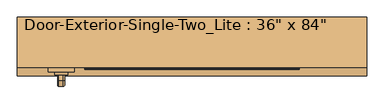
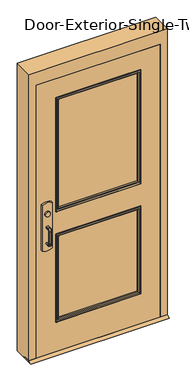
"""IFC4 building model written with IfcOpenShell, lengths in millimetres: door geometry."""

from ifc_helpers import new_model, si_unit, point, frame, frame_2d, origin, place, context, project, spatial, polyline, circle_curve, ellipse_curve, trimmed, segment, composite_curve, outline, extrude, faceted_brep, source, transform, mapped, element, save
from ifc_brep_helpers import plane_surface, cylinder_surface, revolved_surface, advanced_brep


def door_0d86e27c(model_context):
    return source(origin(), model_context, "Body", "SolidModel", [
        extrude(outline(polyline([(-61.9125, 12.7), (-36.5125, 0.0), (-131.7625, 0.0), (-106.3625, 12.7), (-61.9125, 12.7)])), frame((-508.0, 0.0, 0.0), z_axis=(1.0, 0.0, 0.0), x_axis=(0.0, 1.0, 0.0)), (0.0, 0.0, 1.0), 1016.0),
        extrude(outline(polyline([(150.2833333, -23.8125), (150.2833333, -30.1625), (-349.25, -30.1625), (-349.25, -23.8125), (150.2833333, -23.8125)])), frame((0.0, 0.0, 990.6), z_axis=(0.0, 0.0, 1.0), x_axis=(1.0, 0.0, 0.0)), (0.0, 0.0, 1.0), 50.8),
        advanced_brep(
        [(-412.75, -30.1625, 1041.4), (-349.25, -30.1625, 1041.4), (400.05, -30.1625, 1041.4), (400.05, -30.1625, 990.6), (-349.25, -30.1625, 990.6), (-412.75, -30.1625, 990.6), (400.05, -61.9125, 1041.4), (-349.25, -61.9125, 1041.4), (-349.25, -61.9125, 1104.9), (-368.3, -61.9125, 1123.95), (-393.7, -61.9125, 1123.95), (-412.75, -61.9125, 1104.9), (-412.75, -61.9125, 927.1), (-393.7, -61.9125, 908.05), (-368.3, -61.9125, 908.05), (-349.25, -61.9125, 927.1), (-349.25, -61.9125, 990.6), (400.05, -61.9125, 990.6), (-412.75, -33.3377467, 1041.4), (-349.25, -33.3377467, 1041.4), (-412.75, -33.3377467, 990.6), (-412.75, -38.3479269, 927.1), (-412.75, -38.3479269, 1104.9), (-349.25, -33.3377467, 990.6), (-349.25, -38.3479269, 1104.9), (-349.25, -38.3479269, 927.1), (-368.3, -39.850981, 1123.95), (-393.7, -39.850981, 1123.95), (-393.7, -39.850981, 908.05), (-368.3, -39.850981, 908.05)],
        [
            (0, 1),
            (1, 2),
            (2, 3),
            (3, 4),
            (4, 5),
            (5, 0),
            (6, 7),
            (7, 8),
            (8, 9, circle_curve(frame((-368.3, -61.9125, 1104.9), z_axis=(0.0, -1.0, 0.0), x_axis=(1.0, 0.0, 0.0)), 19.05)),
            (9, 10),
            (10, 11, circle_curve(frame((-393.7, -61.9125, 1104.9), z_axis=(0.0, -1.0, 0.0), x_axis=(1.0, 0.0, 0.0)), 19.05)),
            (11, 12),
            (12, 13, circle_curve(frame((-393.7, -61.9125, 927.1), z_axis=(0.0, -1.0, 0.0), x_axis=(1.0, 0.0, 0.0)), 19.05)),
            (13, 14),
            (14, 15, circle_curve(frame((-368.3, -61.9125, 927.1), z_axis=(0.0, -1.0, 0.0), x_axis=(1.0, 0.0, 0.0)), 19.05)),
            (15, 16),
            (16, 17),
            (17, 6),
            (0, 18),
            (18, 19),
            (19, 7),
            (6, 2),
            (5, 20),
            (20, 21),
            (21, 12),
            (11, 22),
            (22, 18),
            (16, 23),
            (23, 20),
            (3, 17),
            (19, 24),
            (24, 8),
            (15, 25),
            (25, 23),
            (9, 26),
            (26, 27),
            (27, 10),
            (13, 28),
            (28, 29),
            (29, 14),
            (29, 25, ellipse_curve(frame((-368.3, -38.3479269, 927.1), z_axis=(0.0, -0.9969018152893365, 0.07865602756830282), x_axis=(0.0, 0.07865602756830208, 0.9969018152893365)), 19.1092038, 19.05)),
            (24, 26, ellipse_curve(frame((-368.3, -38.3479269, 1104.9), z_axis=(0.0, -0.9969018152893376, -0.07865602756828934), x_axis=(0.0, 0.078656027568288, -0.9969018152893377)), 19.1092038, 19.05)),
            (27, 22, ellipse_curve(frame((-393.7, -38.3479269, 1104.9), z_axis=(0.0, -0.9969018152893376, -0.07865602756828934), x_axis=(0.0, 0.078656027568288, -0.9969018152893377)), 19.1092038, 19.05)),
            (21, 28, ellipse_curve(frame((-393.7, -38.3479269, 927.1), z_axis=(0.0, -0.9969018152893365, 0.07865602756830282), x_axis=(0.0, 0.07865602756830208, 0.9969018152893365)), 19.1092038, 19.05)),
        ],
        [
            plane_surface(frame((-412.75, -30.1625, 1041.4), z_axis=(0.0, 1.0, 0.0), x_axis=(-1.0, 0.0, 0.0))),
            plane_surface(frame((-412.75, -61.9125, 1041.4), z_axis=(0.0, -1.0, 0.0), x_axis=(1.0, 0.0, 0.0))),
            plane_surface(frame((400.05, -30.1625, 1041.4), z_axis=(0.0, 0.0, 1.0), x_axis=(0.0, -1.0, 0.0))),
            plane_surface(frame((-412.75, -30.1625, 1041.4), z_axis=(-1.0, 0.0, 0.0), x_axis=(0.0, -1.0, 0.0))),
            plane_surface(frame((-412.75, -30.1625, 990.6), z_axis=(0.0, 0.0, -1.0), x_axis=(0.0, -1.0, 0.0))),
            plane_surface(frame((400.05, -30.1625, 990.6), z_axis=(1.0, 0.0, 0.0), x_axis=(0.0, -1.0, 0.0))),
            plane_surface(frame((-349.25, -33.3377467, 927.1), z_axis=(1.0, 0.0, 0.0), x_axis=(0.0, -1.0, 0.0))),
            plane_surface(frame((-368.3, -33.3377467, 1123.95), z_axis=(0.0, 0.0, 1.0), x_axis=(0.0, -1.0, 0.0))),
            plane_surface(frame((-393.7, -33.3377467, 908.05), z_axis=(0.0, 0.0, -1.0), x_axis=(0.0, -1.0, 0.0))),
            cylinder_surface(frame((-368.3, -61.9125, 927.1), z_axis=(0.0, 1.0, 0.0), x_axis=(1.0, 0.0, 0.0)), 19.05),
            cylinder_surface(frame((-368.3, -61.9125, 1104.9), z_axis=(0.0, 1.0, 0.0), x_axis=(1.0, 0.0, 0.0)), 19.05),
            cylinder_surface(frame((-393.7, -61.9125, 1104.9), z_axis=(0.0, 1.0, 0.0), x_axis=(1.0, 0.0, 0.0)), 19.05),
            cylinder_surface(frame((-393.7, -61.9125, 927.1), z_axis=(0.0, 1.0, 0.0), x_axis=(1.0, 0.0, 0.0)), 19.05),
            plane_surface(frame((-349.25, -33.3377467, 1041.4), z_axis=(0.0, 0.9969018152893376, 0.07865602756828934), x_axis=(-1.0, 0.0, 0.0))),
            plane_surface(frame((-349.25, -39.850981, 908.05), z_axis=(0.0, 0.9969018152893365, -0.07865602756830282), x_axis=(-1.0, 0.0, 0.0))),
        ],
        [
            (0, [[1, 2, 3, 4, 5, 6]]),
            (1, [[7, 8, 9, 10, 11, 12, 13, 14, 15, 16, 17, 18]]),
            (2, [[-2, -1, 19, 20, 21, -7, 22]]),
            (3, [[23, 24, 25, -12, 26, 27, -19, -6]]),
            (4, [[-17, 28, 29, -23, -5, -4, 30]]),
            (5, [[-22, -18, -30, -3]]),
            (6, [[-21, 31, 32, -8]]),
            (6, [[33, 34, -28, -16]]),
            (7, [[35, 36, 37, -10]]),
            (8, [[38, 39, 40, -14]]),
            (9, [[-40, 41, -33, -15]]),
            (10, [[-32, 42, -35, -9]]),
            (11, [[-37, 43, -26, -11]]),
            (12, [[-25, 44, -38, -13]]),
            (13, [[-27, -43, -36, -42, -31, -20]]),
            (14, [[-29, -34, -41, -39, -44, -24]]),
        ],
    ),
        advanced_brep(
        [(-391.0, -119.0625, 1017.190625), (-387.428125, -119.0625, 1020.7625), (-374.571875, -119.0625, 1020.7625), (-371.0, -119.0625, 1017.190625), (-371.0, -119.0625, 1014.8090406), (-374.5715406, -119.0625, 1011.2375), (-387.428125, -119.0625, 1011.2375), (-391.0, -119.0625, 1014.809375), (-391.0, -119.0625, 887.809375), (-391.0, -119.0625, 890.190625), (-387.428125, -119.0625, 893.7625), (-374.5715406, -119.0625, 893.7625), (-371.0, -119.0625, 890.1909594), (-371.0, -119.0625, 887.809375), (-374.571875, -119.0625, 884.2375), (-387.428125, -119.0625, 884.2375), (-391.0, -144.4625, 1014.809375), (-391.0, -155.971875, 1003.3), (-391.0, -155.971875, 901.7), (-391.0, -144.4625, 890.190625), (-391.0, -144.4625, 887.809375), (-391.0, -158.353125, 901.7), (-391.0, -158.353125, 1003.3), (-391.0, -144.4625, 1017.190625), (-387.428125, -144.4625, 1011.2375), (-374.5715406, -144.4625, 1011.2375), (-371.0, -144.4625, 1014.8090406), (-371.0, -144.4625, 1017.190625), (-371.0, -158.353125, 1003.3), (-371.0, -158.353125, 901.7), (-371.0, -144.4625, 887.809375), (-371.0, -144.4625, 890.1909594), (-371.0, -155.9715406, 901.7), (-371.0, -155.9715406, 1003.3), (-374.571875, -144.4625, 1020.7625), (-387.428125, -144.4625, 1020.7625), (-387.428125, -152.4, 1003.3), (-374.5715406, -152.4, 1003.3), (-374.571875, -161.925, 1003.3), (-387.428125, -161.925, 1003.3), (-387.428125, -152.4, 901.7), (-374.5715406, -152.4, 901.7), (-374.571875, -161.925, 901.7), (-387.428125, -161.925, 901.7), (-387.428125, -144.4625, 893.7625), (-374.5715406, -144.4625, 893.7625), (-374.571875, -144.4625, 884.2375), (-387.428125, -144.4625, 884.2375)],
        [
            (0, 1, circle_curve(frame((-387.428125, -119.0625, 1017.190625), z_axis=(0.0, 1.0, 0.0), x_axis=(0.0, 0.0, 1.0)), 3.571875)),
            (1, 2),
            (2, 3, circle_curve(frame((-374.571875, -119.0625, 1017.190625), z_axis=(0.0, 1.0, 0.0), x_axis=(0.0, 0.0, 1.0)), 3.571875)),
            (3, 4),
            (4, 5, circle_curve(frame((-374.5715406, -119.0625, 1014.8090406), z_axis=(0.0, 1.0, 0.0), x_axis=(0.0, 0.0, 1.0)), 3.5715406)),
            (5, 6),
            (6, 7, circle_curve(frame((-387.428125, -119.0625, 1014.809375), z_axis=(0.0, 1.0, 0.0), x_axis=(0.0, 0.0, 1.0)), 3.571875)),
            (7, 0),
            (8, 9),
            (9, 10, circle_curve(frame((-387.428125, -119.0625, 890.190625), z_axis=(0.0, 1.0, 0.0), x_axis=(0.0, 0.0, -1.0)), 3.571875)),
            (10, 11),
            (11, 12, circle_curve(frame((-374.5715406, -119.0625, 890.1909594), z_axis=(0.0, 1.0, 0.0), x_axis=(0.0, 0.0, -1.0)), 3.5715406)),
            (12, 13),
            (13, 14, circle_curve(frame((-374.571875, -119.0625, 887.809375), z_axis=(0.0, 1.0, 0.0), x_axis=(0.0, 0.0, -1.0)), 3.571875)),
            (14, 15),
            (15, 8, circle_curve(frame((-387.428125, -119.0625, 887.809375), z_axis=(0.0, 1.0, 0.0), x_axis=(0.0, 0.0, -1.0)), 3.571875)),
            (7, 16),
            (16, 17, circle_curve(frame((-391.0, -144.4625, 1003.3), z_axis=(1.0, 0.0, 0.0), x_axis=(0.0, 0.0, 1.0)), 11.509375)),
            (17, 18),
            (18, 19, circle_curve(frame((-391.0, -144.4625, 901.7), z_axis=(1.0, 0.0, 0.0), x_axis=(0.0, -1.0, 0.0)), 11.509375)),
            (19, 9),
            (8, 20),
            (20, 21, circle_curve(frame((-391.0, -144.4625, 901.7), z_axis=(-1.0, 0.0, 0.0), x_axis=(0.0, -1.0, 0.0)), 13.890625)),
            (21, 22),
            (22, 23, circle_curve(frame((-391.0, -144.4625, 1003.3), z_axis=(-1.0, 0.0, 0.0), x_axis=(0.0, 0.0, 1.0)), 13.890625)),
            (23, 0),
            (6, 24),
            (24, 16, circle_curve(frame((-387.428125, -144.4625, 1014.809375), z_axis=(0.0, 1.0, 0.0), x_axis=(0.0, 0.0, 1.0)), 3.571875)),
            (5, 25),
            (25, 24),
            (4, 26),
            (26, 25, circle_curve(frame((-374.5715406, -144.4625, 1014.8090406), z_axis=(0.0, 1.0, 0.0), x_axis=(0.0, 0.0, 1.0)), 3.5715406)),
            (3, 27),
            (27, 28, circle_curve(frame((-371.0, -144.4625, 1003.3), z_axis=(1.0, 0.0, 0.0), x_axis=(0.0, 0.0, 1.0)), 13.890625)),
            (28, 29),
            (29, 30, circle_curve(frame((-371.0, -144.4625, 901.7), z_axis=(1.0, 0.0, 0.0), x_axis=(0.0, -1.0, 0.0)), 13.890625)),
            (30, 13),
            (12, 31),
            (31, 32, circle_curve(frame((-371.0, -144.4625, 901.7), z_axis=(-1.0, 0.0, 0.0), x_axis=(0.0, -1.0, 0.0)), 11.5090406)),
            (32, 33),
            (33, 26, circle_curve(frame((-371.0, -144.4625, 1003.3), z_axis=(-1.0, 0.0, 0.0), x_axis=(0.0, 0.0, 1.0)), 11.5090406)),
            (2, 34),
            (34, 27, circle_curve(frame((-374.571875, -144.4625, 1017.190625), z_axis=(0.0, 1.0, 0.0), x_axis=(0.0, 0.0, 1.0)), 3.571875)),
            (1, 35),
            (35, 34),
            (23, 35, circle_curve(frame((-387.428125, -144.4625, 1017.190625), z_axis=(0.0, 1.0, 0.0), x_axis=(0.0, 0.0, 1.0)), 3.571875)),
            (36, 17, circle_curve(frame((-387.428125, -155.971875, 1003.3), z_axis=(0.0, 0.0, 1.0), x_axis=(0.0, -1.0, 0.0)), 3.571875)),
            (24, 36, circle_curve(frame((-387.428125, -144.4625, 1003.3), z_axis=(1.0, 0.0, 0.0), x_axis=(0.0, 0.0, 1.0)), 7.9375)),
            (37, 36),
            (25, 37, circle_curve(frame((-374.5715406, -144.4625, 1003.3), z_axis=(1.0, 0.0, 0.0), x_axis=(0.0, 0.0, 1.0)), 7.9375)),
            (33, 37, circle_curve(frame((-374.5715406, -155.9715406, 1003.3), z_axis=(0.0, 0.0, 1.0), x_axis=(0.0, -1.0, 0.0)), 3.5715406)),
            (38, 28, circle_curve(frame((-374.571875, -158.353125, 1003.3), z_axis=(0.0, 0.0, 1.0), x_axis=(0.0, -1.0, 0.0)), 3.571875)),
            (34, 38, circle_curve(frame((-374.571875, -144.4625, 1003.3), z_axis=(1.0, 0.0, 0.0), x_axis=(0.0, 0.0, 1.0)), 17.4625)),
            (39, 38),
            (35, 39, circle_curve(frame((-387.428125, -144.4625, 1003.3), z_axis=(1.0, 0.0, 0.0), x_axis=(0.0, 0.0, 1.0)), 17.4625)),
            (22, 39, circle_curve(frame((-387.428125, -158.353125, 1003.3), z_axis=(0.0, 0.0, 1.0), x_axis=(0.0, -1.0, 0.0)), 3.571875)),
            (36, 40),
            (40, 18, circle_curve(frame((-387.428125, -155.971875, 901.7), z_axis=(0.0, 0.0, 1.0), x_axis=(0.0, -1.0, 0.0)), 3.571875)),
            (37, 41),
            (41, 40),
            (32, 41, circle_curve(frame((-374.5715406, -155.9715406, 901.7), z_axis=(0.0, 0.0, 1.0), x_axis=(0.0, -1.0, 0.0)), 3.5715406)),
            (38, 42),
            (42, 29, circle_curve(frame((-374.571875, -158.353125, 901.7), z_axis=(0.0, 0.0, 1.0), x_axis=(0.0, -1.0, 0.0)), 3.571875)),
            (39, 43),
            (43, 42),
            (21, 43, circle_curve(frame((-387.428125, -158.353125, 901.7), z_axis=(0.0, 0.0, 1.0), x_axis=(0.0, -1.0, 0.0)), 3.571875)),
            (44, 19, circle_curve(frame((-387.428125, -144.4625, 890.190625), z_axis=(0.0, -1.0, 0.0), x_axis=(0.0, 0.0, -1.0)), 3.571875)),
            (40, 44, circle_curve(frame((-387.428125, -144.4625, 901.7), z_axis=(1.0, 0.0, 0.0), x_axis=(0.0, -1.0, 0.0)), 7.9375)),
            (45, 44),
            (41, 45, circle_curve(frame((-374.5715406, -144.4625, 901.7), z_axis=(1.0, 0.0, 0.0), x_axis=(0.0, -1.0, 0.0)), 7.9375)),
            (31, 45, circle_curve(frame((-374.5715406, -144.4625, 890.1909594), z_axis=(0.0, -1.0, 0.0), x_axis=(0.0, 0.0, -1.0)), 3.5715406)),
            (46, 30, circle_curve(frame((-374.571875, -144.4625, 887.809375), z_axis=(0.0, -1.0, 0.0), x_axis=(0.0, 0.0, -1.0)), 3.571875)),
            (42, 46, circle_curve(frame((-374.571875, -144.4625, 901.7), z_axis=(1.0, 0.0, 0.0), x_axis=(0.0, -1.0, 0.0)), 17.4625)),
            (47, 46),
            (43, 47, circle_curve(frame((-387.428125, -144.4625, 901.7), z_axis=(1.0, 0.0, 0.0), x_axis=(0.0, -1.0, 0.0)), 17.4625)),
            (20, 47, circle_curve(frame((-387.428125, -144.4625, 887.809375), z_axis=(0.0, -1.0, 0.0), x_axis=(0.0, 0.0, -1.0)), 3.571875)),
            (44, 10),
            (45, 11),
            (46, 14),
            (47, 15),
        ],
        [
            plane_surface(frame((-381.0, -119.0625, 1016.0), z_axis=(0.0, 1.0, 0.0), x_axis=(1.0, 0.0, 0.0))),
            plane_surface(frame((-381.0, -119.0625, 889.0), z_axis=(0.0, 1.0, 0.0), x_axis=(1.0, 0.0, 0.0))),
            plane_surface(frame((-391.0, -119.0625, 1017.190625), z_axis=(-1.0, 0.0, 0.0), x_axis=(0.0, -1.0, 0.0))),
            cylinder_surface(frame((-387.428125, -119.0625, 1014.809375), z_axis=(0.0, 1.0, 0.0), x_axis=(0.0, 0.0, 1.0)), 3.571875),
            plane_surface(frame((-387.428125, -119.0625, 1011.2375), z_axis=(0.0, 0.0, -1.0), x_axis=(0.0, -1.0, 0.0))),
            cylinder_surface(frame((-374.5715406, -119.0625, 1014.8090406), z_axis=(0.0, 1.0, 0.0), x_axis=(0.0, 0.0, 1.0)), 3.5715406),
            plane_surface(frame((-371.0, -119.0625, 1014.8090406), z_axis=(1.0, 0.0, 0.0), x_axis=(0.0, -1.0, 0.0))),
            cylinder_surface(frame((-374.571875, -119.0625, 1017.190625), z_axis=(0.0, 1.0, 0.0), x_axis=(0.0, 0.0, 1.0)), 3.571875),
            plane_surface(frame((-374.571875, -119.0625, 1020.7625), z_axis=(0.0, 0.0, 1.0), x_axis=(0.0, -1.0, 0.0))),
            cylinder_surface(frame((-387.428125, -119.0625, 1017.190625), z_axis=(0.0, 1.0, 0.0), x_axis=(0.0, 0.0, 1.0)), 3.571875),
            revolved_surface(trimmed(ellipse_curve(frame((-387.428125, -144.4625, 1014.809375), z_axis=(0.0, -1.0, 0.0), x_axis=(0.0, 0.0, 1.0)), 3.571875, 3.571875), [point((-391.0, -144.4625, 1014.809375))], [point((-387.428125, -144.4625, 1011.2375))], True, "CARTESIAN"), (-381.0, -144.4625, 1003.3), (-1.0, 0.0, 0.0)),
            revolved_surface(polyline([(-387.428125, -144.4625, 1011.2375), (-374.5715406, -144.4625, 1011.2375)]), (-381.0, -144.4625, 1003.3), (-1.0, 0.0, 0.0)),
            revolved_surface(trimmed(ellipse_curve(frame((-374.5715406, -144.4625, 1014.8090406), z_axis=(0.0, -1.0, 0.0), x_axis=(0.0, 0.0, 1.0)), 3.5715406, 3.5715406), [point((-374.5715406, -144.4625, 1011.2375))], [point((-371.0, -144.4625, 1014.8090406))], True, "CARTESIAN"), (-381.0, -144.4625, 1003.3), (-1.0, 0.0, 0.0)),
            revolved_surface(trimmed(ellipse_curve(frame((-374.571875, -144.4625, 1017.190625), z_axis=(0.0, -1.0, 0.0), x_axis=(0.0, 0.0, 1.0)), 3.571875, 3.571875), [point((-371.0, -144.4625, 1017.190625))], [point((-374.571875, -144.4625, 1020.7625))], True, "CARTESIAN"), (-381.0, -144.4625, 1003.3), (-1.0, 0.0, 0.0)),
            cylinder_surface(frame((-381.0, -144.4625, 1003.3), z_axis=(-1.0, 0.0, 0.0), x_axis=(0.0, 0.0, 1.0)), 17.4625),
            revolved_surface(trimmed(ellipse_curve(frame((-387.428125, -144.4625, 1017.190625), z_axis=(0.0, -1.0, 0.0), x_axis=(0.0, 0.0, 1.0)), 3.571875, 3.571875), [point((-387.428125, -144.4625, 1020.7625))], [point((-391.0, -144.4625, 1017.190625))], True, "CARTESIAN"), (-381.0, -144.4625, 1003.3), (-1.0, 0.0, 0.0)),
            cylinder_surface(frame((-387.428125, -155.971875, 1003.3), z_axis=(0.0, 0.0, 1.0), x_axis=(0.0, -1.0, 0.0)), 3.571875),
            plane_surface(frame((-387.428125, -152.4, 1003.3), z_axis=(0.0, 1.0, 0.0), x_axis=(0.0, 0.0, -1.0))),
            cylinder_surface(frame((-374.5715406, -155.9715406, 1003.3), z_axis=(0.0, 0.0, 1.0), x_axis=(0.0, -1.0, 0.0)), 3.5715406),
            cylinder_surface(frame((-374.571875, -158.353125, 1003.3), z_axis=(0.0, 0.0, 1.0), x_axis=(0.0, -1.0, 0.0)), 3.571875),
            plane_surface(frame((-374.571875, -161.925, 1003.3), z_axis=(0.0, -1.0, 0.0), x_axis=(0.0, 0.0, -1.0))),
            cylinder_surface(frame((-387.428125, -158.353125, 1003.3), z_axis=(0.0, 0.0, 1.0), x_axis=(0.0, -1.0, 0.0)), 3.571875),
            revolved_surface(trimmed(ellipse_curve(frame((-387.428125, -155.971875, 901.7), z_axis=(0.0, 0.0, -1.0), x_axis=(0.0, -1.0, 0.0)), 3.571875, 3.571875), [point((-391.0, -155.971875, 901.7))], [point((-387.428125, -152.4, 901.7))], True, "CARTESIAN"), (-381.0, -144.4625, 901.7), (-1.0, 0.0, 0.0)),
            revolved_surface(polyline([(-387.428125, -152.4, 901.7), (-374.5715406, -152.4, 901.7)]), (-381.0, -144.4625, 901.7), (-1.0, 0.0, 0.0)),
            revolved_surface(trimmed(ellipse_curve(frame((-374.5715406, -155.9715406, 901.7), z_axis=(0.0, 0.0, -1.0), x_axis=(0.0, -1.0, 0.0)), 3.5715406, 3.5715406), [point((-374.5715406, -152.4, 901.7))], [point((-371.0, -155.9715406, 901.7))], True, "CARTESIAN"), (-381.0, -144.4625, 901.7), (-1.0, 0.0, 0.0)),
            revolved_surface(trimmed(ellipse_curve(frame((-374.571875, -158.353125, 901.7), z_axis=(0.0, 0.0, -1.0), x_axis=(0.0, -1.0, 0.0)), 3.571875, 3.571875), [point((-371.0, -158.353125, 901.7))], [point((-374.571875, -161.925, 901.7))], True, "CARTESIAN"), (-381.0, -144.4625, 901.7), (-1.0, 0.0, 0.0)),
            cylinder_surface(frame((-381.0, -144.4625, 901.7), z_axis=(-1.0, 0.0, 0.0), x_axis=(0.0, -1.0, 0.0)), 17.4625),
            revolved_surface(trimmed(ellipse_curve(frame((-387.428125, -158.353125, 901.7), z_axis=(0.0, 0.0, -1.0), x_axis=(0.0, -1.0, 0.0)), 3.571875, 3.571875), [point((-387.428125, -161.925, 901.7))], [point((-391.0, -158.353125, 901.7))], True, "CARTESIAN"), (-381.0, -144.4625, 901.7), (-1.0, 0.0, 0.0)),
            cylinder_surface(frame((-387.428125, -144.4625, 890.190625), z_axis=(0.0, -1.0, 0.0), x_axis=(0.0, 0.0, -1.0)), 3.571875),
            plane_surface(frame((-387.428125, -144.4625, 893.7625), z_axis=(0.0, 0.0, 1.0), x_axis=(0.0, 1.0, 0.0))),
            cylinder_surface(frame((-374.5715406, -144.4625, 890.1909594), z_axis=(0.0, -1.0, 0.0), x_axis=(0.0, 0.0, -1.0)), 3.5715406),
            cylinder_surface(frame((-374.571875, -144.4625, 887.809375), z_axis=(0.0, -1.0, 0.0), x_axis=(0.0, 0.0, -1.0)), 3.571875),
            plane_surface(frame((-374.571875, -144.4625, 884.2375), z_axis=(0.0, 0.0, -1.0), x_axis=(0.0, 1.0, 0.0))),
            cylinder_surface(frame((-387.428125, -144.4625, 887.809375), z_axis=(0.0, -1.0, 0.0), x_axis=(0.0, 0.0, -1.0)), 3.571875),
        ],
        [
            (0, [[1, 2, 3, 4, 5, 6, 7, 8]]),
            (1, [[9, 10, 11, 12, 13, 14, 15, 16]]),
            (2, [[17, 18, 19, 20, 21, -9, 22, 23, 24, 25, 26, -8]]),
            (3, [[27, 28, -17, -7]]),
            (4, [[29, 30, -27, -6]]),
            (5, [[31, 32, -29, -5]]),
            (6, [[33, 34, 35, 36, 37, -13, 38, 39, 40, 41, -31, -4]]),
            (7, [[42, 43, -33, -3]]),
            (8, [[44, 45, -42, -2]]),
            (9, [[-26, 46, -44, -1]]),
            (10, [[47, -18, -28, 48]]),
            (11, [[49, -48, -30, 50]]),
            (12, [[51, -50, -32, -41]]),
            (13, [[52, -34, -43, 53]]),
            (14, [[54, -53, -45, 55]]),
            (15, [[56, -55, -46, -25]]),
            (16, [[57, 58, -19, -47]]),
            (17, [[59, 60, -57, -49]]),
            (18, [[-40, 61, -59, -51]]),
            (19, [[62, 63, -35, -52]]),
            (20, [[64, 65, -62, -54]]),
            (21, [[-24, 66, -64, -56]]),
            (22, [[67, -20, -58, 68]]),
            (23, [[69, -68, -60, 70]]),
            (24, [[71, -70, -61, -39]]),
            (25, [[72, -36, -63, 73]]),
            (26, [[74, -73, -65, 75]]),
            (27, [[76, -75, -66, -23]]),
            (28, [[77, -10, -21, -67]]),
            (29, [[78, -11, -77, -69]]),
            (30, [[-38, -12, -78, -71]]),
            (31, [[79, -14, -37, -72]]),
            (32, [[80, -15, -79, -74]]),
            (33, [[-22, -16, -80, -76]]),
        ],
    ),
        extrude(outline(composite_curve([segment(trimmed(circle_curve(frame_2d((1117.6, -381.0)), 19.0), [point((1117.6, -400.0))], [point((1117.6, -362.0))], False, "CARTESIAN"), True, "CONTINUOUS"), segment(trimmed(circle_curve(frame_2d((1117.6, -381.0)), 19.0), [point((1117.6, -362.0))], [point((1117.6, -400.0))], False, "CARTESIAN"), True, "CONTINUOUS")], self_intersect=False)), frame((0.0, -127.79375, 0.0), z_axis=(0.0, 1.0, 0.0), x_axis=(0.0, 0.0, 1.0)), (0.0, 0.0, 1.0), 8.73125),
        extrude(outline(composite_curve([segment(trimmed(circle_curve(frame_2d((1113.0338574, -381.0)), 89.3016225), [point((1193.8, -342.9))], [point((1193.8, -419.1))], False, "CARTESIAN"), True, "CONTINUOUS"), segment(polyline([(1193.8, -419.1), (838.2, -419.1)]), True, "CONTINUOUS"), segment(trimmed(circle_curve(frame_2d((918.9661426, -381.0)), 89.3016225), [point((838.2, -419.1))], [point((838.2, -342.9))], False, "CARTESIAN"), True, "CONTINUOUS"), segment(polyline([(838.2, -342.9), (1193.8, -342.9)]), True, "CONTINUOUS")], self_intersect=False)), frame((0.0, -119.0625, 0.0), z_axis=(0.0, 1.0, 0.0), x_axis=(0.0, 0.0, 1.0)), (0.0, 0.0, 1.0), 12.7),
        faceted_brep([(457.2, -57.15, 0.0), (441.325, -57.15, 0.0), (441.325, -9.525, 0.0), (457.2, -9.525, 0.0), (457.2, 39.6875, 0.0), (508.0, 39.6875, 0.0), (508.0, -106.3625, 0.0), (457.2, -106.3625, 0.0), (457.2, -106.3625, 2133.6), (457.2, -57.15, 2133.6), (508.0, -106.3625, 2235.2), (-508.0, -106.3625, 2235.2), (-508.0, -106.3625, 0.0), (-457.2, -106.3625, 0.0), (-457.2, -106.3625, 2133.6), (508.0, 39.6875, 2235.2), (457.2, 39.6875, 2133.6), (-457.2, 39.6875, 2133.6), (-457.2, 39.6875, 0.0), (-508.0, 39.6875, 0.0), (-508.0, 39.6875, 2235.2), (457.2, -9.525, 2133.6), (441.325, -9.525, 2117.725), (-441.325, -9.525, 2117.725), (-441.325, -9.525, 0.0), (-457.2, -9.525, 0.0), (-457.2, -9.525, 2133.6), (441.325, -57.15, 2117.725), (-457.2, -57.15, 2133.6), (-457.2, -57.15, 0.0), (-441.325, -57.15, 0.0), (-441.325, -57.15, 2117.725)], [[[0, 1, 2, 3, 4, 5, 6, 7]], [[7, 8, 9, 0]], [[6, 10, 11, 12, 13, 14, 8, 7]], [[5, 15, 10, 6]], [[4, 16, 17, 18, 19, 20, 15, 5]], [[3, 21, 16, 4]], [[2, 22, 23, 24, 25, 26, 21, 3]], [[1, 27, 22, 2]], [[0, 9, 28, 29, 30, 31, 27, 1]], [[8, 14, 28, 9]], [[16, 21, 26, 17]], [[22, 27, 31, 23]], [[12, 19, 18, 25, 24, 30, 29, 13]], [[13, 29, 28, 14]], [[11, 20, 19, 12]], [[17, 26, 25, 18]], [[23, 31, 30, 24]], [[15, 20, 11, 10]]]),
        extrude(outline(polyline([(2133.6, -457.2), (12.7, -457.2), (12.7, 457.2), (2133.6, 457.2), (2133.6, -457.2)]), holes=[polyline([(1981.2, -304.8), (1981.2, 304.8), (1111.25, 304.8), (1111.25, -304.8), (1981.2, -304.8)]), polyline([(920.75, -304.8), (920.75, 304.8), (254.0, 304.8), (254.0, -304.8), (920.75, -304.8)])]), frame((0.0, -106.3625, 0.0), z_axis=(0.0, 1.0, 0.0), x_axis=(0.0, 0.0, 1.0)), (0.0, 0.0, 1.0), 44.45),
        extrude(outline(polyline([(304.8, -74.6125), (304.8, -93.6625), (-304.8, -93.6625), (-304.8, -74.6125), (304.8, -74.6125)])), frame((0.0, 0.0, 1111.25), z_axis=(0.0, 0.0, 1.0), x_axis=(1.0, 0.0, 0.0)), (0.0, 0.0, 1.0), 869.95),
        extrude(outline(polyline([(304.8, -74.6125), (304.8, -93.6625), (-304.8, -93.6625), (-304.8, -74.6125), (304.8, -74.6125)])), frame((0.0, 0.0, 254.0), z_axis=(0.0, 0.0, 1.0), x_axis=(1.0, 0.0, 0.0)), (0.0, 0.0, 1.0), 666.75),
        advanced_brep(
        [(304.8, -74.6125, 920.75), (304.8, -74.6125, 254.0), (304.8, -61.9125, 254.0), (304.8, -61.9125, 920.75), (292.8, -60.9125, 908.75), (292.8, -60.9125, 266.0), (292.8, -74.6125, 266.0), (292.8, -74.6125, 908.75), (297.8, -55.9125, 913.75), (297.8, -55.9125, 261.0), (312.8, -57.9125, 928.75), (312.8, -57.9125, 246.0), (310.8, -55.9125, 248.0), (310.8, -55.9125, 926.75), (312.8, -61.9125, 928.75), (312.8, -61.9125, 246.0), (-304.8, -74.6125, 254.0), (-304.8, -61.9125, 254.0), (-292.8, -60.9125, 266.0), (-292.8, -74.6125, 266.0), (-297.8, -55.9125, 261.0), (-312.8, -57.9125, 246.0), (-310.8, -55.9125, 248.0), (-312.8, -61.9125, 246.0), (-304.8, -74.6125, 920.75), (-304.8, -61.9125, 920.75), (-292.8, -60.9125, 908.75), (-292.8, -74.6125, 908.75), (-297.8, -55.9125, 913.75), (-312.8, -57.9125, 928.75), (-310.8, -55.9125, 926.75), (-312.8, -61.9125, 928.75)],
        [
            (0, 1),
            (1, 2),
            (2, 3),
            (3, 0),
            (4, 5),
            (5, 6),
            (6, 7),
            (7, 4),
            (8, 9),
            (9, 5, ellipse_curve(frame((297.8, -60.9125, 261.0), z_axis=(0.7071067811865475, 0.0, 0.7071067811865475), x_axis=(-0.7071067811865474, 0.0, 0.7071067811865476)), 7.0710678, 5.0)),
            (4, 8, ellipse_curve(frame((297.8, -60.9125, 913.75), z_axis=(0.7071067811865475, 0.0, -0.7071067811865475), x_axis=(0.7071067811865474, 0.0, 0.7071067811865476)), 7.0710678, 5.0)),
            (10, 11),
            (11, 12, ellipse_curve(frame((310.8, -57.9125, 248.0), z_axis=(0.7071067811865475, 0.0, 0.7071067811865475), x_axis=(-0.7071067811865474, 0.0, 0.7071067811865476)), 2.8284271, 2.0)),
            (12, 13),
            (13, 10, ellipse_curve(frame((310.8, -57.9125, 926.75), z_axis=(0.7071067811865475, 0.0, -0.7071067811865475), x_axis=(0.7071067811865474, 0.0, 0.7071067811865476)), 2.8284271, 2.0)),
            (14, 15),
            (15, 11),
            (10, 14),
            (1, 16),
            (16, 17),
            (17, 2),
            (5, 18),
            (18, 19),
            (19, 6),
            (9, 20),
            (20, 18, ellipse_curve(frame((-297.8, -60.9125, 261.0), z_axis=(0.7071067811865475, 0.0, -0.7071067811865475), x_axis=(0.7071067811865476, 0.0, 0.7071067811865474)), 7.0710678, 5.0)),
            (11, 21),
            (21, 22, ellipse_curve(frame((-310.8, -57.9125, 248.0), z_axis=(0.7071067811865475, 0.0, -0.7071067811865475), x_axis=(0.7071067811865476, 0.0, 0.7071067811865474)), 2.8284271, 2.0)),
            (22, 12),
            (15, 23),
            (23, 21),
            (16, 24),
            (24, 25),
            (25, 17),
            (18, 26),
            (26, 27),
            (27, 19),
            (20, 28),
            (28, 26, ellipse_curve(frame((-297.8, -60.9125, 913.75), z_axis=(-0.7071067811865475, 0.0, -0.7071067811865475), x_axis=(0.7071067811865474, 0.0, -0.7071067811865476)), 7.0710678, 5.0)),
            (21, 29),
            (29, 30, ellipse_curve(frame((-310.8, -57.9125, 926.75), z_axis=(-0.7071067811865475, 0.0, -0.7071067811865475), x_axis=(0.7071067811865474, 0.0, -0.7071067811865476)), 2.8284271, 2.0)),
            (30, 22),
            (23, 31),
            (31, 29),
            (14, 31),
            (25, 3),
            (24, 0),
            (27, 7),
            (26, 4),
            (28, 8),
            (30, 13),
            (29, 10),
        ],
        [
            plane_surface(frame((304.8, -61.9125, 920.75), z_axis=(1.0, 0.0, 0.0), x_axis=(0.0, 0.0, -1.0))),
            plane_surface(frame((292.8, -74.6125, 908.75), z_axis=(-1.0, 0.0, 0.0), x_axis=(0.0, 0.0, -1.0))),
            cylinder_surface(frame((297.8, -60.9125, 920.75), z_axis=(0.0, 0.0, 1.0), x_axis=(1.0, 0.0, 0.0)), 5.0),
            cylinder_surface(frame((310.8, -57.9125, 920.75), z_axis=(0.0, 0.0, 1.0), x_axis=(1.0, 0.0, 0.0)), 2.0),
            plane_surface(frame((312.8, -57.9125, 928.75), z_axis=(1.0, 0.0, 0.0), x_axis=(0.0, 0.0, -1.0))),
            plane_surface(frame((304.8, -61.9125, 254.0), z_axis=(0.0, 0.0, -1.0), x_axis=(-1.0, 0.0, 0.0))),
            plane_surface(frame((292.8, -74.6125, 266.0), z_axis=(0.0, 0.0, 1.0), x_axis=(-1.0, 0.0, 0.0))),
            cylinder_surface(frame((304.8, -60.9125, 261.0), z_axis=(1.0, 0.0, 0.0), x_axis=(0.0, 0.0, -1.0)), 5.0),
            cylinder_surface(frame((304.8, -57.9125, 248.0), z_axis=(1.0, 0.0, 0.0), x_axis=(0.0, 0.0, -1.0)), 2.0),
            plane_surface(frame((312.8, -57.9125, 246.0), z_axis=(0.0, 0.0, -1.0), x_axis=(-1.0, 0.0, 0.0))),
            plane_surface(frame((-304.8, -61.9125, 254.0), z_axis=(-1.0, 0.0, 0.0), x_axis=(0.0, 0.0, 1.0))),
            plane_surface(frame((-292.8, -74.6125, 266.0), z_axis=(1.0, 0.0, 0.0), x_axis=(0.0, 0.0, 1.0))),
            cylinder_surface(frame((-297.8, -60.9125, 254.0), z_axis=(0.0, 0.0, -1.0), x_axis=(-1.0, 0.0, 0.0)), 5.0),
            cylinder_surface(frame((-310.8, -57.9125, 254.0), z_axis=(0.0, 0.0, -1.0), x_axis=(-1.0, 0.0, 0.0)), 2.0),
            plane_surface(frame((-312.8, -57.9125, 246.0), z_axis=(-1.0, 0.0, 0.0), x_axis=(0.0, 0.0, 1.0))),
            plane_surface(frame((-312.8, -61.9125, 928.75), z_axis=(0.0, -1.0, 0.0), x_axis=(1.0, 0.0, 0.0))),
            plane_surface(frame((-304.8, -61.9125, 920.75), z_axis=(0.0, 0.0, 1.0), x_axis=(1.0, 0.0, 0.0))),
            plane_surface(frame((-304.8, -74.6125, 920.75), z_axis=(0.0, -1.0, 0.0), x_axis=(1.0, 0.0, 0.0))),
            plane_surface(frame((-292.8, -74.6125, 908.75), z_axis=(0.0, 0.0, -1.0), x_axis=(1.0, 0.0, 0.0))),
            cylinder_surface(frame((-304.8, -60.9125, 913.75), z_axis=(-1.0, 0.0, 0.0), x_axis=(0.0, 0.0, 1.0)), 5.0),
            plane_surface(frame((-297.8, -55.9125, 913.75), z_axis=(0.0, 1.0, 0.0), x_axis=(1.0, 0.0, 0.0))),
            cylinder_surface(frame((-304.8, -57.9125, 926.75), z_axis=(-1.0, 0.0, 0.0), x_axis=(0.0, 0.0, 1.0)), 2.0),
            plane_surface(frame((-312.8, -57.9125, 928.75), z_axis=(0.0, 0.0, 1.0), x_axis=(1.0, 0.0, 0.0))),
        ],
        [
            (0, [[1, 2, 3, 4]]),
            (1, [[5, 6, 7, 8]]),
            (2, [[9, 10, -5, 11]]),
            (3, [[12, 13, 14, 15]]),
            (4, [[16, 17, -12, 18]]),
            (5, [[19, 20, 21, -2]]),
            (6, [[22, 23, 24, -6]]),
            (7, [[25, 26, -22, -10]]),
            (8, [[27, 28, 29, -13]]),
            (9, [[30, 31, -27, -17]]),
            (10, [[32, 33, 34, -20]]),
            (11, [[35, 36, 37, -23]]),
            (12, [[38, 39, -35, -26]]),
            (13, [[40, 41, 42, -28]]),
            (14, [[43, 44, -40, -31]]),
            (15, [[-16, 45, -43, -30], [-3, -21, -34, 46]]),
            (16, [[47, -4, -46, -33]]),
            (17, [[-1, -47, -32, -19], [-7, -24, -37, 48]]),
            (18, [[49, -8, -48, -36]]),
            (19, [[50, -11, -49, -39]]),
            (20, [[-14, -29, -42, 51], [-9, -50, -38, -25]]),
            (21, [[52, -15, -51, -41]]),
            (22, [[-45, -18, -52, -44]]),
        ],
    ),
        advanced_brep(
        [(-304.8, -93.6625, 920.75), (-304.8, -93.6625, 254.0), (-304.8, -106.3625, 254.0), (-304.8, -106.3625, 920.75), (-292.8, -107.3625, 908.75), (-292.8, -107.3625, 266.0), (-292.8, -93.6625, 266.0), (-292.8, -93.6625, 908.75), (-297.8, -112.3625, 913.75), (-297.8, -112.3625, 261.0), (-312.8, -110.3625, 928.75), (-312.8, -110.3625, 246.0), (-310.8, -112.3625, 248.0), (-310.8, -112.3625, 926.75), (-312.8, -106.3625, 928.75), (-312.8, -106.3625, 246.0), (304.8, -93.6625, 254.0), (304.8, -106.3625, 254.0), (292.8, -107.3625, 266.0), (292.8, -93.6625, 266.0), (297.8, -112.3625, 261.0), (312.8, -110.3625, 246.0), (310.8, -112.3625, 248.0), (312.8, -106.3625, 246.0), (304.8, -93.6625, 920.75), (304.8, -106.3625, 920.75), (292.8, -107.3625, 908.75), (292.8, -93.6625, 908.75), (297.8, -112.3625, 913.75), (312.8, -110.3625, 928.75), (310.8, -112.3625, 926.75), (312.8, -106.3625, 928.75)],
        [
            (0, 1),
            (1, 2),
            (2, 3),
            (3, 0),
            (4, 5),
            (5, 6),
            (6, 7),
            (7, 4),
            (8, 9),
            (9, 5, ellipse_curve(frame((-297.8, -107.3625, 261.0), z_axis=(-0.7071067811865475, 0.0, 0.7071067811865475), x_axis=(0.7071067811865474, 0.0, 0.7071067811865476)), 7.0710678, 5.0)),
            (4, 8, ellipse_curve(frame((-297.8, -107.3625, 913.75), z_axis=(-0.7071067811865475, 0.0, -0.7071067811865475), x_axis=(-0.7071067811865474, 0.0, 0.7071067811865476)), 7.0710678, 5.0)),
            (10, 11),
            (11, 12, ellipse_curve(frame((-310.8, -110.3625, 248.0), z_axis=(-0.7071067811865475, 0.0, 0.7071067811865475), x_axis=(0.7071067811865474, 0.0, 0.7071067811865476)), 2.8284271, 2.0)),
            (12, 13),
            (13, 10, ellipse_curve(frame((-310.8, -110.3625, 926.75), z_axis=(-0.7071067811865475, 0.0, -0.7071067811865475), x_axis=(-0.7071067811865474, 0.0, 0.7071067811865476)), 2.8284271, 2.0)),
            (14, 15),
            (15, 11),
            (10, 14),
            (1, 16),
            (16, 17),
            (17, 2),
            (5, 18),
            (18, 19),
            (19, 6),
            (9, 20),
            (20, 18, ellipse_curve(frame((297.8, -107.3625, 261.0), z_axis=(-0.7071067811865475, 0.0, -0.7071067811865475), x_axis=(-0.7071067811865476, 0.0, 0.7071067811865474)), 7.0710678, 5.0)),
            (11, 21),
            (21, 22, ellipse_curve(frame((310.8, -110.3625, 248.0), z_axis=(-0.7071067811865475, 0.0, -0.7071067811865475), x_axis=(-0.7071067811865476, 0.0, 0.7071067811865474)), 2.8284271, 2.0)),
            (22, 12),
            (15, 23),
            (23, 21),
            (16, 24),
            (24, 25),
            (25, 17),
            (18, 26),
            (26, 27),
            (27, 19),
            (20, 28),
            (28, 26, ellipse_curve(frame((297.8, -107.3625, 913.75), z_axis=(0.7071067811865475, 0.0, -0.7071067811865475), x_axis=(-0.7071067811865474, 0.0, -0.7071067811865476)), 7.0710678, 5.0)),
            (21, 29),
            (29, 30, ellipse_curve(frame((310.8, -110.3625, 926.75), z_axis=(0.7071067811865475, 0.0, -0.7071067811865475), x_axis=(-0.7071067811865474, 0.0, -0.7071067811865476)), 2.8284271, 2.0)),
            (30, 22),
            (23, 31),
            (31, 29),
            (14, 31),
            (25, 3),
            (24, 0),
            (27, 7),
            (26, 4),
            (28, 8),
            (30, 13),
            (29, 10),
        ],
        [
            plane_surface(frame((-304.8, -106.3625, 920.75), z_axis=(-1.0, 0.0, 0.0), x_axis=(0.0, 0.0, -1.0))),
            plane_surface(frame((-292.8, -93.6625, 908.75), z_axis=(1.0, 0.0, 0.0), x_axis=(0.0, 0.0, -1.0))),
            cylinder_surface(frame((-297.8, -107.3625, 920.75), z_axis=(0.0, 0.0, 1.0), x_axis=(-1.0, 0.0, 0.0)), 5.0),
            cylinder_surface(frame((-310.8, -110.3625, 920.75), z_axis=(0.0, 0.0, 1.0), x_axis=(-1.0, 0.0, 0.0)), 2.0),
            plane_surface(frame((-312.8, -110.3625, 928.75), z_axis=(-1.0, 0.0, 0.0), x_axis=(0.0, 0.0, -1.0))),
            plane_surface(frame((-304.8, -106.3625, 254.0), z_axis=(0.0, 0.0, -1.0), x_axis=(1.0, 0.0, 0.0))),
            plane_surface(frame((-292.8, -93.6625, 266.0), z_axis=(0.0, 0.0, 1.0), x_axis=(1.0, 0.0, 0.0))),
            cylinder_surface(frame((-304.8, -107.3625, 261.0), z_axis=(-1.0, 0.0, 0.0), x_axis=(0.0, 0.0, -1.0)), 5.0),
            cylinder_surface(frame((-304.8, -110.3625, 248.0), z_axis=(-1.0, 0.0, 0.0), x_axis=(0.0, 0.0, -1.0)), 2.0),
            plane_surface(frame((-312.8, -110.3625, 246.0), z_axis=(0.0, 0.0, -1.0), x_axis=(1.0, 0.0, 0.0))),
            plane_surface(frame((304.8, -106.3625, 254.0), z_axis=(1.0, 0.0, 0.0), x_axis=(0.0, 0.0, 1.0))),
            plane_surface(frame((292.8, -93.6625, 266.0), z_axis=(-1.0, 0.0, 0.0), x_axis=(0.0, 0.0, 1.0))),
            cylinder_surface(frame((297.8, -107.3625, 254.0), z_axis=(0.0, 0.0, -1.0), x_axis=(1.0, 0.0, 0.0)), 5.0),
            cylinder_surface(frame((310.8, -110.3625, 254.0), z_axis=(0.0, 0.0, -1.0), x_axis=(1.0, 0.0, 0.0)), 2.0),
            plane_surface(frame((312.8, -110.3625, 246.0), z_axis=(1.0, 0.0, 0.0), x_axis=(0.0, 0.0, 1.0))),
            plane_surface(frame((312.8, -106.3625, 928.75), z_axis=(0.0, 1.0, 0.0), x_axis=(-1.0, 0.0, 0.0))),
            plane_surface(frame((304.8, -106.3625, 920.75), z_axis=(0.0, 0.0, 1.0), x_axis=(-1.0, 0.0, 0.0))),
            plane_surface(frame((304.8, -93.6625, 920.75), z_axis=(0.0, 1.0, 0.0), x_axis=(-1.0, 0.0, 0.0))),
            plane_surface(frame((292.8, -93.6625, 908.75), z_axis=(0.0, 0.0, -1.0), x_axis=(-1.0, 0.0, 0.0))),
            cylinder_surface(frame((304.8, -107.3625, 913.75), z_axis=(1.0, 0.0, 0.0), x_axis=(0.0, 0.0, 1.0)), 5.0),
            plane_surface(frame((297.8, -112.3625, 913.75), z_axis=(0.0, -1.0, 0.0), x_axis=(-1.0, 0.0, 0.0))),
            cylinder_surface(frame((304.8, -110.3625, 926.75), z_axis=(1.0, 0.0, 0.0), x_axis=(0.0, 0.0, 1.0)), 2.0),
            plane_surface(frame((312.8, -110.3625, 928.75), z_axis=(0.0, 0.0, 1.0), x_axis=(-1.0, 0.0, 0.0))),
        ],
        [
            (0, [[1, 2, 3, 4]]),
            (1, [[5, 6, 7, 8]]),
            (2, [[9, 10, -5, 11]]),
            (3, [[12, 13, 14, 15]]),
            (4, [[16, 17, -12, 18]]),
            (5, [[19, 20, 21, -2]]),
            (6, [[22, 23, 24, -6]]),
            (7, [[25, 26, -22, -10]]),
            (8, [[27, 28, 29, -13]]),
            (9, [[30, 31, -27, -17]]),
            (10, [[32, 33, 34, -20]]),
            (11, [[35, 36, 37, -23]]),
            (12, [[38, 39, -35, -26]]),
            (13, [[40, 41, 42, -28]]),
            (14, [[43, 44, -40, -31]]),
            (15, [[-16, 45, -43, -30], [-3, -21, -34, 46]]),
            (16, [[47, -4, -46, -33]]),
            (17, [[-1, -47, -32, -19], [-7, -24, -37, 48]]),
            (18, [[49, -8, -48, -36]]),
            (19, [[50, -11, -49, -39]]),
            (20, [[-14, -29, -42, 51], [-9, -50, -38, -25]]),
            (21, [[52, -15, -51, -41]]),
            (22, [[-45, -18, -52, -44]]),
        ],
    ),
        advanced_brep(
        [(-304.8, -74.6125, 1111.25), (-304.8, -74.6125, 1981.2), (-304.8, -61.9125, 1981.2), (-304.8, -61.9125, 1111.25), (-292.8, -60.9125, 1123.25), (-292.8, -60.9125, 1969.2), (-292.8, -74.6125, 1969.2), (-292.8, -74.6125, 1123.25), (-297.8, -55.9125, 1118.25), (-297.8, -55.9125, 1974.2), (-312.8, -57.9125, 1103.25), (-312.8, -57.9125, 1989.2), (-310.8, -55.9125, 1987.2), (-310.8, -55.9125, 1105.25), (-312.8, -61.9125, 1103.25), (-312.8, -61.9125, 1989.2), (304.8, -74.6125, 1981.2), (304.8, -61.9125, 1981.2), (292.8, -60.9125, 1969.2), (292.8, -74.6125, 1969.2), (297.8, -55.9125, 1974.2), (312.8, -57.9125, 1989.2), (310.8, -55.9125, 1987.2), (312.8, -61.9125, 1989.2), (304.8, -74.6125, 1111.25), (304.8, -61.9125, 1111.25), (292.8, -60.9125, 1123.25), (292.8, -74.6125, 1123.25), (297.8, -55.9125, 1118.25), (312.8, -57.9125, 1103.25), (310.8, -55.9125, 1105.25), (312.8, -61.9125, 1103.25)],
        [
            (0, 1),
            (1, 2),
            (2, 3),
            (3, 0),
            (4, 5),
            (5, 6),
            (6, 7),
            (7, 4),
            (8, 9),
            (9, 5, ellipse_curve(frame((-297.8, -60.9125, 1974.2), z_axis=(-0.7071067811865475, 0.0, -0.7071067811865475), x_axis=(0.7071067811865474, 0.0, -0.7071067811865476)), 7.0710678, 5.0)),
            (4, 8, ellipse_curve(frame((-297.8, -60.9125, 1118.25), z_axis=(-0.7071067811865475, 0.0, 0.7071067811865475), x_axis=(-0.7071067811865474, 0.0, -0.7071067811865476)), 7.0710678, 5.0)),
            (10, 11),
            (11, 12, ellipse_curve(frame((-310.8, -57.9125, 1987.2), z_axis=(-0.7071067811865475, 0.0, -0.7071067811865475), x_axis=(0.7071067811865474, 0.0, -0.7071067811865476)), 2.8284271, 2.0)),
            (12, 13),
            (13, 10, ellipse_curve(frame((-310.8, -57.9125, 1105.25), z_axis=(-0.7071067811865475, 0.0, 0.7071067811865475), x_axis=(-0.7071067811865474, 0.0, -0.7071067811865476)), 2.8284271, 2.0)),
            (14, 15),
            (15, 11),
            (10, 14),
            (1, 16),
            (16, 17),
            (17, 2),
            (5, 18),
            (18, 19),
            (19, 6),
            (9, 20),
            (20, 18, ellipse_curve(frame((297.8, -60.9125, 1974.2), z_axis=(-0.7071067811865475, 0.0, 0.7071067811865475), x_axis=(-0.7071067811865476, 0.0, -0.7071067811865474)), 7.0710678, 5.0)),
            (11, 21),
            (21, 22, ellipse_curve(frame((310.8, -57.9125, 1987.2), z_axis=(-0.7071067811865475, 0.0, 0.7071067811865475), x_axis=(-0.7071067811865476, 0.0, -0.7071067811865474)), 2.8284271, 2.0)),
            (22, 12),
            (15, 23),
            (23, 21),
            (16, 24),
            (24, 25),
            (25, 17),
            (18, 26),
            (26, 27),
            (27, 19),
            (20, 28),
            (28, 26, ellipse_curve(frame((297.8, -60.9125, 1118.25), z_axis=(0.7071067811865475, 0.0, 0.7071067811865475), x_axis=(-0.7071067811865474, 0.0, 0.7071067811865476)), 7.0710678, 5.0)),
            (21, 29),
            (29, 30, ellipse_curve(frame((310.8, -57.9125, 1105.25), z_axis=(0.7071067811865475, 0.0, 0.7071067811865475), x_axis=(-0.7071067811865474, 0.0, 0.7071067811865476)), 2.8284271, 2.0)),
            (30, 22),
            (23, 31),
            (31, 29),
            (14, 31),
            (25, 3),
            (24, 0),
            (27, 7),
            (26, 4),
            (28, 8),
            (30, 13),
            (29, 10),
        ],
        [
            plane_surface(frame((-304.8, -61.9125, 1111.25), z_axis=(-1.0, 0.0, 0.0), x_axis=(0.0, 0.0, 1.0))),
            plane_surface(frame((-292.8, -74.6125, 1123.25), z_axis=(1.0, 0.0, 0.0), x_axis=(0.0, 0.0, 1.0))),
            cylinder_surface(frame((-297.8, -60.9125, 1111.25), z_axis=(0.0, 0.0, -1.0), x_axis=(-1.0, 0.0, 0.0)), 5.0),
            cylinder_surface(frame((-310.8, -57.9125, 1111.25), z_axis=(0.0, 0.0, -1.0), x_axis=(-1.0, 0.0, 0.0)), 2.0),
            plane_surface(frame((-312.8, -57.9125, 1103.25), z_axis=(-1.0, 0.0, 0.0), x_axis=(0.0, 0.0, 1.0))),
            plane_surface(frame((-304.8, -61.9125, 1981.2), z_axis=(0.0, 0.0, 1.0), x_axis=(1.0, 0.0, 0.0))),
            plane_surface(frame((-292.8, -74.6125, 1969.2), z_axis=(0.0, 0.0, -1.0), x_axis=(1.0, 0.0, 0.0))),
            cylinder_surface(frame((-304.8, -60.9125, 1974.2), z_axis=(-1.0, 0.0, 0.0), x_axis=(0.0, 0.0, 1.0)), 5.0),
            cylinder_surface(frame((-304.8, -57.9125, 1987.2), z_axis=(-1.0, 0.0, 0.0), x_axis=(0.0, 0.0, 1.0)), 2.0),
            plane_surface(frame((-312.8, -57.9125, 1989.2), z_axis=(0.0, 0.0, 1.0), x_axis=(1.0, 0.0, 0.0))),
            plane_surface(frame((304.8, -61.9125, 1981.2), z_axis=(1.0, 0.0, 0.0), x_axis=(0.0, 0.0, -1.0))),
            plane_surface(frame((292.8, -74.6125, 1969.2), z_axis=(-1.0, 0.0, 0.0), x_axis=(0.0, 0.0, -1.0))),
            cylinder_surface(frame((297.8, -60.9125, 1981.2), z_axis=(0.0, 0.0, 1.0), x_axis=(1.0, 0.0, 0.0)), 5.0),
            cylinder_surface(frame((310.8, -57.9125, 1981.2), z_axis=(0.0, 0.0, 1.0), x_axis=(1.0, 0.0, 0.0)), 2.0),
            plane_surface(frame((312.8, -57.9125, 1989.2), z_axis=(1.0, 0.0, 0.0), x_axis=(0.0, 0.0, -1.0))),
            plane_surface(frame((312.8, -61.9125, 1103.25), z_axis=(0.0, -1.0, 0.0), x_axis=(-1.0, 0.0, 0.0))),
            plane_surface(frame((304.8, -61.9125, 1111.25), z_axis=(0.0, 0.0, -1.0), x_axis=(-1.0, 0.0, 0.0))),
            plane_surface(frame((304.8, -74.6125, 1111.25), z_axis=(0.0, -1.0, 0.0), x_axis=(-1.0, 0.0, 0.0))),
            plane_surface(frame((292.8, -74.6125, 1123.25), z_axis=(0.0, 0.0, 1.0), x_axis=(-1.0, 0.0, 0.0))),
            cylinder_surface(frame((304.8, -60.9125, 1118.25), z_axis=(1.0, 0.0, 0.0), x_axis=(0.0, 0.0, -1.0)), 5.0),
            plane_surface(frame((297.8, -55.9125, 1118.25), z_axis=(0.0, 1.0, 0.0), x_axis=(-1.0, 0.0, 0.0))),
            cylinder_surface(frame((304.8, -57.9125, 1105.25), z_axis=(1.0, 0.0, 0.0), x_axis=(0.0, 0.0, -1.0)), 2.0),
            plane_surface(frame((312.8, -57.9125, 1103.25), z_axis=(0.0, 0.0, -1.0), x_axis=(-1.0, 0.0, 0.0))),
        ],
        [
            (0, [[1, 2, 3, 4]]),
            (1, [[5, 6, 7, 8]]),
            (2, [[9, 10, -5, 11]]),
            (3, [[12, 13, 14, 15]]),
            (4, [[16, 17, -12, 18]]),
            (5, [[19, 20, 21, -2]]),
            (6, [[22, 23, 24, -6]]),
            (7, [[25, 26, -22, -10]]),
            (8, [[27, 28, 29, -13]]),
            (9, [[30, 31, -27, -17]]),
            (10, [[32, 33, 34, -20]]),
            (11, [[35, 36, 37, -23]]),
            (12, [[38, 39, -35, -26]]),
            (13, [[40, 41, 42, -28]]),
            (14, [[43, 44, -40, -31]]),
            (15, [[-16, 45, -43, -30], [-3, -21, -34, 46]]),
            (16, [[47, -4, -46, -33]]),
            (17, [[-1, -47, -32, -19], [-7, -24, -37, 48]]),
            (18, [[49, -8, -48, -36]]),
            (19, [[50, -11, -49, -39]]),
            (20, [[-14, -29, -42, 51], [-9, -50, -38, -25]]),
            (21, [[52, -15, -51, -41]]),
            (22, [[-45, -18, -52, -44]]),
        ],
    ),
        advanced_brep(
        [(-304.8, -93.6625, 1981.2), (-304.8, -93.6625, 1111.25), (-304.8, -106.3625, 1111.25), (-304.8, -106.3625, 1981.2), (-292.8, -107.3625, 1969.2), (-292.8, -107.3625, 1123.25), (-292.8, -93.6625, 1123.25), (-292.8, -93.6625, 1969.2), (-297.8, -112.3625, 1974.2), (-297.8, -112.3625, 1118.25), (-312.8, -110.3625, 1989.2), (-312.8, -110.3625, 1103.25), (-310.8, -112.3625, 1105.25), (-310.8, -112.3625, 1987.2), (-312.8, -106.3625, 1989.2), (-312.8, -106.3625, 1103.25), (304.8, -93.6625, 1111.25), (304.8, -106.3625, 1111.25), (292.8, -107.3625, 1123.25), (292.8, -93.6625, 1123.25), (297.8, -112.3625, 1118.25), (312.8, -110.3625, 1103.25), (310.8, -112.3625, 1105.25), (312.8, -106.3625, 1103.25), (304.8, -93.6625, 1981.2), (304.8, -106.3625, 1981.2), (292.8, -107.3625, 1969.2), (292.8, -93.6625, 1969.2), (297.8, -112.3625, 1974.2), (312.8, -110.3625, 1989.2), (310.8, -112.3625, 1987.2), (312.8, -106.3625, 1989.2)],
        [
            (0, 1),
            (1, 2),
            (2, 3),
            (3, 0),
            (4, 5),
            (5, 6),
            (6, 7),
            (7, 4),
            (8, 9),
            (9, 5, ellipse_curve(frame((-297.8, -107.3625, 1118.25), z_axis=(-0.7071067811865475, 0.0, 0.7071067811865475), x_axis=(0.7071067811865474, 0.0, 0.7071067811865476)), 7.0710678, 5.0)),
            (4, 8, ellipse_curve(frame((-297.8, -107.3625, 1974.2), z_axis=(-0.7071067811865475, 0.0, -0.7071067811865475), x_axis=(-0.7071067811865474, 0.0, 0.7071067811865476)), 7.0710678, 5.0)),
            (10, 11),
            (11, 12, ellipse_curve(frame((-310.8, -110.3625, 1105.25), z_axis=(-0.7071067811865475, 0.0, 0.7071067811865475), x_axis=(0.7071067811865474, 0.0, 0.7071067811865476)), 2.8284271, 2.0)),
            (12, 13),
            (13, 10, ellipse_curve(frame((-310.8, -110.3625, 1987.2), z_axis=(-0.7071067811865475, 0.0, -0.7071067811865475), x_axis=(-0.7071067811865474, 0.0, 0.7071067811865476)), 2.8284271, 2.0)),
            (14, 15),
            (15, 11),
            (10, 14),
            (1, 16),
            (16, 17),
            (17, 2),
            (5, 18),
            (18, 19),
            (19, 6),
            (9, 20),
            (20, 18, ellipse_curve(frame((297.8, -107.3625, 1118.25), z_axis=(-0.7071067811865475, 0.0, -0.7071067811865475), x_axis=(-0.7071067811865476, 0.0, 0.7071067811865474)), 7.0710678, 5.0)),
            (11, 21),
            (21, 22, ellipse_curve(frame((310.8, -110.3625, 1105.25), z_axis=(-0.7071067811865475, 0.0, -0.7071067811865475), x_axis=(-0.7071067811865476, 0.0, 0.7071067811865474)), 2.8284271, 2.0)),
            (22, 12),
            (15, 23),
            (23, 21),
            (16, 24),
            (24, 25),
            (25, 17),
            (18, 26),
            (26, 27),
            (27, 19),
            (20, 28),
            (28, 26, ellipse_curve(frame((297.8, -107.3625, 1974.2), z_axis=(0.7071067811865475, 0.0, -0.7071067811865475), x_axis=(-0.7071067811865474, 0.0, -0.7071067811865476)), 7.0710678, 5.0)),
            (21, 29),
            (29, 30, ellipse_curve(frame((310.8, -110.3625, 1987.2), z_axis=(0.7071067811865475, 0.0, -0.7071067811865475), x_axis=(-0.7071067811865474, 0.0, -0.7071067811865476)), 2.8284271, 2.0)),
            (30, 22),
            (23, 31),
            (31, 29),
            (14, 31),
            (25, 3),
            (24, 0),
            (27, 7),
            (26, 4),
            (28, 8),
            (30, 13),
            (29, 10),
        ],
        [
            plane_surface(frame((-304.8, -106.3625, 1981.2), z_axis=(-1.0, 0.0, 0.0), x_axis=(0.0, 0.0, -1.0))),
            plane_surface(frame((-292.8, -93.6625, 1969.2), z_axis=(1.0, 0.0, 0.0), x_axis=(0.0, 0.0, -1.0))),
            cylinder_surface(frame((-297.8, -107.3625, 1981.2), z_axis=(0.0, 0.0, 1.0), x_axis=(-1.0, 0.0, 0.0)), 5.0),
            cylinder_surface(frame((-310.8, -110.3625, 1981.2), z_axis=(0.0, 0.0, 1.0), x_axis=(-1.0, 0.0, 0.0)), 2.0),
            plane_surface(frame((-312.8, -110.3625, 1989.2), z_axis=(-1.0, 0.0, 0.0), x_axis=(0.0, 0.0, -1.0))),
            plane_surface(frame((-304.8, -106.3625, 1111.25), z_axis=(0.0, 0.0, -1.0), x_axis=(1.0, 0.0, 0.0))),
            plane_surface(frame((-292.8, -93.6625, 1123.25), z_axis=(0.0, 0.0, 1.0), x_axis=(1.0, 0.0, 0.0))),
            cylinder_surface(frame((-304.8, -107.3625, 1118.25), z_axis=(-1.0, 0.0, 0.0), x_axis=(0.0, 0.0, -1.0)), 5.0),
            cylinder_surface(frame((-304.8, -110.3625, 1105.25), z_axis=(-1.0, 0.0, 0.0), x_axis=(0.0, 0.0, -1.0)), 2.0),
            plane_surface(frame((-312.8, -110.3625, 1103.25), z_axis=(0.0, 0.0, -1.0), x_axis=(1.0, 0.0, 0.0))),
            plane_surface(frame((304.8, -106.3625, 1111.25), z_axis=(1.0, 0.0, 0.0), x_axis=(0.0, 0.0, 1.0))),
            plane_surface(frame((292.8, -93.6625, 1123.25), z_axis=(-1.0, 0.0, 0.0), x_axis=(0.0, 0.0, 1.0))),
            cylinder_surface(frame((297.8, -107.3625, 1111.25), z_axis=(0.0, 0.0, -1.0), x_axis=(1.0, 0.0, 0.0)), 5.0),
            cylinder_surface(frame((310.8, -110.3625, 1111.25), z_axis=(0.0, 0.0, -1.0), x_axis=(1.0, 0.0, 0.0)), 2.0),
            plane_surface(frame((312.8, -110.3625, 1103.25), z_axis=(1.0, 0.0, 0.0), x_axis=(0.0, 0.0, 1.0))),
            plane_surface(frame((312.8, -106.3625, 1989.2), z_axis=(0.0, 1.0, 0.0), x_axis=(-1.0, 0.0, 0.0))),
            plane_surface(frame((304.8, -106.3625, 1981.2), z_axis=(0.0, 0.0, 1.0), x_axis=(-1.0, 0.0, 0.0))),
            plane_surface(frame((304.8, -93.6625, 1981.2), z_axis=(0.0, 1.0, 0.0), x_axis=(-1.0, 0.0, 0.0))),
            plane_surface(frame((292.8, -93.6625, 1969.2), z_axis=(0.0, 0.0, -1.0), x_axis=(-1.0, 0.0, 0.0))),
            cylinder_surface(frame((304.8, -107.3625, 1974.2), z_axis=(1.0, 0.0, 0.0), x_axis=(0.0, 0.0, 1.0)), 5.0),
            plane_surface(frame((297.8, -112.3625, 1974.2), z_axis=(0.0, -1.0, 0.0), x_axis=(-1.0, 0.0, 0.0))),
            cylinder_surface(frame((304.8, -110.3625, 1987.2), z_axis=(1.0, 0.0, 0.0), x_axis=(0.0, 0.0, 1.0)), 2.0),
            plane_surface(frame((312.8, -110.3625, 1989.2), z_axis=(0.0, 0.0, 1.0), x_axis=(-1.0, 0.0, 0.0))),
        ],
        [
            (0, [[1, 2, 3, 4]]),
            (1, [[5, 6, 7, 8]]),
            (2, [[9, 10, -5, 11]]),
            (3, [[12, 13, 14, 15]]),
            (4, [[16, 17, -12, 18]]),
            (5, [[19, 20, 21, -2]]),
            (6, [[22, 23, 24, -6]]),
            (7, [[25, 26, -22, -10]]),
            (8, [[27, 28, 29, -13]]),
            (9, [[30, 31, -27, -17]]),
            (10, [[32, 33, 34, -20]]),
            (11, [[35, 36, 37, -23]]),
            (12, [[38, 39, -35, -26]]),
            (13, [[40, 41, 42, -28]]),
            (14, [[43, 44, -40, -31]]),
            (15, [[-16, 45, -43, -30], [-3, -21, -34, 46]]),
            (16, [[47, -4, -46, -33]]),
            (17, [[-1, -47, -32, -19], [-7, -24, -37, 48]]),
            (18, [[49, -8, -48, -36]]),
            (19, [[50, -11, -49, -39]]),
            (20, [[-14, -29, -42, 51], [-9, -50, -38, -25]]),
            (21, [[52, -15, -51, -41]]),
            (22, [[-45, -18, -52, -44]]),
        ],
    ),
    ])


if __name__ == "__main__":
    model = new_model("IFC4")
    model_context = context("Model", 3, world=origin())
    ifc_project = project(units=[si_unit("LENGTHUNIT", "METRE", prefix="MILLI")], contexts=[model_context])
    site = spatial("IfcSite", under=ifc_project)
    building = spatial("IfcBuilding", under=site)
    placement = place(None, origin())
    door_shape = door_0d86e27c(model_context)
    element("IfcDoor", 1, ObjectType="Door-Exterior-Single-Two_Lite : 36\" x 84\"", at=placement, inside=building, context=model_context, shape_type="MappedRepresentation", body=[
        mapped(door_shape, transform((0.0, 0.0, 0.0), x_axis=(1.0, 0.0, 0.0), y_axis=(0.0, 1.0, 0.0), z_axis=(0.0, 0.0, 1.0))),
    ])
    save(model, "model.ifc")

# Revit data of these elements
# Type "Door-Exterior-Single-Two_Lite : 36\" x 84\""
#   Type Mark = "24"
#   Assembly Code = "B2030100"
#   Analytic Construction = "Metal frame, double glass door"
#   Top Rail = 0' - 6"
#   Threshold Offset [instance default] = 0' - 0 1/2"
#   Threshold Length [instance default] = 3' - 4"
#   Thickness = 0' - 1 3/4"
#   Thermal Resistance (R) = 1.3794 (h·ft²·°F)/BTU
#   Swing Angle [instance default] = 90.00°
#   Strike Height = 3' - 4"
#   Stiles = 0' - 6"
#   Rough Width [instance default] = 3' - 4"
#   Rough Height [instance default] = 7' - 4"
#   MFOpeningHeight [instance default] = 0' - 4"
#   MFOpeningWidth [instance default] = 0' - 4"
#   Lock Rail = 0' - 7 1/2"
#   Heat Transfer Coefficient (U) = 0.7250 BTU/(h·ft²·°F)
#   Glass Thickness = 0' - 0 3/4"
#   Inset Calculate [instance default] = 0' - 4"
#   Masonry Inset [instance default] = 0' - 1"
#   Height = 7' - 0"
#   Width = 3' - 0"
#   Masonry Frame Depth = 0' - 5 3/4"
#   Bottom Rail = 0' - 10"
#   Function = 0
#   Masonry Frame [instance default] = yes
#   Function = 1
#   Threshold [instance default] = yes
#   Dry Wall Frame [instance default] = no
#   Threshold Material = none
#   Panic Bar Material = Metal - Stainless Steel
#   Panel Material = Metal - Painted - Grey
#   Glass Stop Material = Metal - Painted - Grey
#   Exterior Pull Material = Metal - Stainless Steel
#   Frame Material = Metal - Painted - Grey
#   Visual Light Transmittance = 0
#   Solar Heat Gain Coefficient = 0
#   Wall Closure = (empty or 0)
# Element 1 (IfcDoor, "Door-Exterior-Single-Two_Lite : 36\" x 84\"")
#   Inset Calculate = 0' - 8"
#   Masonry Inset = 0' - 5"
#   Materials on its faces: "Metal - Painted - Grey", "Metal - Stainless Steel", "Glass"
# Materials
#   "Metal - Stainless Steel": class "Metal", colour RGB 247 247 247, transparency 0
#   "Metal - Painted - Grey": class "Paint", colour RGB 104 104 104, transparency 0
#   "Glass": class "Unassigned", colour RGB 0 128 192, transparency 0.75, Description = "Glass"
